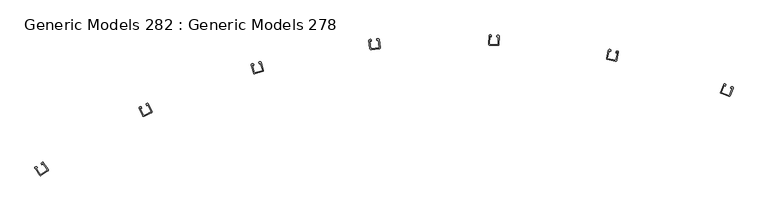
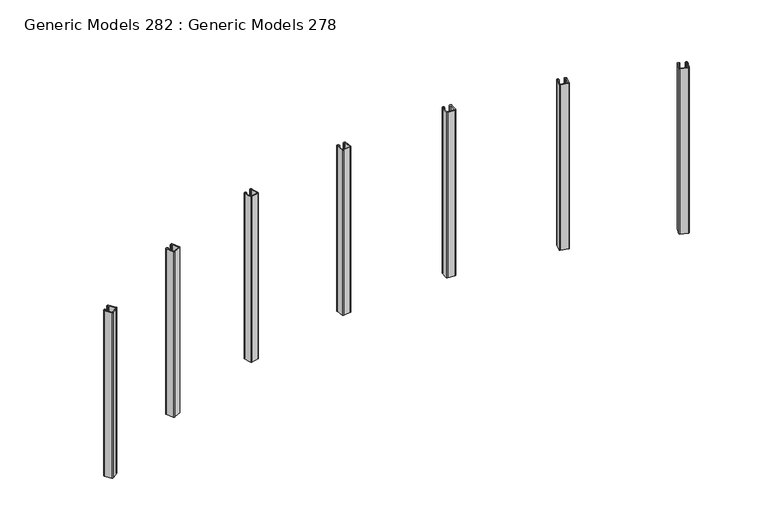
"""IFC4 building model written with IfcOpenShell, lengths in millimetres: proxy geometry, Generic Models 282 : Generic Models 278."""

from ifc_helpers import new_model, si_unit, point, frame, frame_2d, origin, place, context, project, spatial, polyline, circle_curve, trimmed, segment, composite_curve, outline, extrude, source, transform, mapped, element, save


def generic_models_282_generic_models_278_72c7d637(model_context):
    return source(origin(), model_context, "Body", "SweptSolid", [
        extrude(outline(composite_curve([segment(trimmed(circle_curve(frame_2d((271.5326409, -22367.9486308)), 3.9532868), [point((267.8419297, -22366.5318995))], [point((272.9493722, -22364.2579196))], False, "CARTESIAN"), True, "CONTINUOUS"), segment(polyline([(272.9493722, -22364.2579196), (274.3929251, -22364.8120477)]), True, "CONTINUOUS"), segment(trimmed(circle_curve(frame_2d((272.9503297, -22368.5701372)), 4.0254588), [point((274.3929251, -22364.8120477))], [point((276.7084192, -22370.0127326))], False, "CARTESIAN"), True, "CONTINUOUS"), segment(polyline([(276.7084192, -22370.0127326), (264.8013944, -22401.0315926)]), True, "CONTINUOUS"), segment(trimmed(circle_curve(frame_2d((261.0448118, -22399.5895756)), 4.0238446), [point((264.8013944, -22401.0315926))], [point((259.6027949, -22403.3461582))], False, "CARTESIAN"), True, "CONTINUOUS"), segment(polyline([(259.6027949, -22403.3461582), (228.5455312, -22391.4243917)]), True, "CONTINUOUS"), segment(trimmed(circle_curve(frame_2d((229.9733849, -22387.7047058)), 3.9843229), [point((228.5455312, -22391.4243917))], [point((226.253699, -22386.2768522))], False, "CARTESIAN"), True, "CONTINUOUS"), segment(polyline([(226.253699, -22386.2768522), (238.1797429, -22355.2084456)]), True, "CONTINUOUS"), segment(trimmed(circle_curve(frame_2d((241.9251825, -22356.6461852)), 4.0119089), [point((238.1797429, -22355.2084456))], [point((243.3629221, -22352.9007455))], False, "CARTESIAN"), True, "CONTINUOUS"), segment(polyline([(243.3629221, -22352.9007455), (244.734154, -22353.4271121)]), True, "CONTINUOUS"), segment(trimmed(circle_curve(frame_2d((243.2848054, -22357.2027942)), 4.0443029), [point((244.734154, -22353.4271121))], [point((247.0604875, -22358.6521427))], False, "CARTESIAN"), True, "CONTINUOUS"), segment(polyline([(247.0604875, -22358.6521427), (245.949745, -22361.5457259), (242.9856271, -22360.4079076), (244.0963696, -22357.5143245)]), True, "CONTINUOUS"), segment(trimmed(circle_curve(frame_2d((243.2848054, -22357.2027942)), 0.8693029), [point((244.0963696, -22357.5143245))], [point((243.5963357, -22356.39123))], True, "CARTESIAN"), True, "CONTINUOUS"), segment(polyline([(243.5963357, -22356.39123), (242.2251039, -22355.8648634)]), True, "CONTINUOUS"), segment(trimmed(circle_curve(frame_2d((241.9251825, -22356.6461852)), 0.8369089), [point((242.2251039, -22355.8648634))], [point((241.1438607, -22356.3462638))], True, "CARTESIAN"), True, "CONTINUOUS"), segment(polyline([(241.1438607, -22356.3462638), (229.2178168, -22387.4146704)]), True, "CONTINUOUS"), segment(trimmed(circle_curve(frame_2d((229.9733849, -22387.7047058)), 0.8093229), [point((229.2178168, -22387.4146704))], [point((229.6833495, -22388.4602738))], True, "CARTESIAN"), True, "CONTINUOUS"), segment(polyline([(229.6833495, -22388.4602738), (260.7406131, -22400.3820404)]), True, "CONTINUOUS"), segment(trimmed(circle_curve(frame_2d((261.0448118, -22399.5895756)), 0.8488446), [point((260.7406131, -22400.3820404))], [point((261.8372765, -22399.8937744))], True, "CARTESIAN"), True, "CONTINUOUS"), segment(polyline([(261.8372765, -22399.8937744), (273.7443013, -22368.8749143)]), True, "CONTINUOUS"), segment(trimmed(circle_curve(frame_2d((272.9503297, -22368.5701372)), 0.8504588), [point((273.7443013, -22368.8749143))], [point((273.2551068, -22367.7761655))], True, "CARTESIAN"), True, "CONTINUOUS"), segment(polyline([(273.2551068, -22367.7761655), (271.8115539, -22367.2220375)]), True, "CONTINUOUS"), segment(trimmed(circle_curve(frame_2d((271.5326409, -22367.9486308)), 0.7782868), [point((271.8115539, -22367.2220375))], [point((270.8060476, -22367.6697178))], True, "CARTESIAN"), True, "CONTINUOUS"), segment(polyline([(270.8060476, -22367.6697178), (269.6626878, -22370.6482718), (266.69857, -22369.5104535), (267.8419297, -22366.5318995)]), True, "CONTINUOUS")], self_intersect=False)), frame((0.0, 0.0, 203.2), z_axis=(0.0, 0.0, 1.0), x_axis=(1.0, 0.0, 0.0)), (0.0, 0.0, 1.0), 790.575),
        extrude(outline(composite_curve([segment(trimmed(circle_curve(frame_2d((-192.9016412, -22223.7493173)), 3.9532868), [point((-196.7670988, -22222.920635))], [point((-192.0729589, -22219.8838598))], False, "CARTESIAN"), True, "CONTINUOUS"), segment(polyline([(-192.0729589, -22219.8838598), (-190.5610572, -22220.2079834)]), True, "CONTINUOUS"), segment(trimmed(circle_curve(frame_2d((-191.4048681, -22224.1440095)), 4.0254588), [point((-190.5610572, -22220.2079834))], [point((-187.468842, -22224.9878204))], False, "CARTESIAN"), True, "CONTINUOUS"), segment(polyline([(-187.468842, -22224.9878204), (-194.4335648, -22257.4753496)]), True, "CONTINUOUS"), segment(trimmed(circle_curve(frame_2d((-198.3680126, -22256.6318771)), 4.0238446), [point((-194.4335648, -22257.4753496))], [point((-199.2114852, -22260.5663249))], False, "CARTESIAN"), True, "CONTINUOUS"), segment(polyline([(-199.2114852, -22260.5663249), (-231.7392362, -22253.5929793)]), True, "CONTINUOUS"), segment(trimmed(circle_curve(frame_2d((-230.9040482, -22249.6971751)), 3.9843229), [point((-231.7392362, -22253.5929793))], [point((-234.7998524, -22248.8619871))], False, "CARTESIAN"), True, "CONTINUOUS"), segment(polyline([(-234.7998524, -22248.8619871), (-227.8240048, -22216.3225654)]), True, "CONTINUOUS"), segment(trimmed(circle_curve(frame_2d((-223.9012275, -22217.163536)), 4.0119089), [point((-227.8240048, -22216.3225654))], [point((-223.060257, -22213.2407587))], False, "CARTESIAN"), True, "CONTINUOUS"), segment(polyline([(-223.060257, -22213.2407587), (-221.6241005, -22213.548644)]), True, "CONTINUOUS"), segment(trimmed(circle_curve(frame_2d((-222.4718615, -22217.5030956)), 4.0443029), [point((-221.6241005, -22213.548644))], [point((-218.5174099, -22218.3508565))], False, "CARTESIAN"), True, "CONTINUOUS"), segment(polyline([(-218.5174099, -22218.3508565), (-219.1671115, -22221.3814439), (-222.2715733, -22220.715905), (-221.6218717, -22217.6853176)]), True, "CONTINUOUS"), segment(trimmed(circle_curve(frame_2d((-222.4718615, -22217.5030956)), 0.8693029), [point((-221.6218717, -22217.6853176))], [point((-222.2896394, -22216.6531058))], True, "CARTESIAN"), True, "CONTINUOUS"), segment(polyline([(-222.2896394, -22216.6531058), (-223.7257959, -22216.3452205)]), True, "CONTINUOUS"), segment(trimmed(circle_curve(frame_2d((-223.9012275, -22217.163536)), 0.8369089), [point((-223.7257959, -22216.3452205))], [point((-224.719543, -22216.9881044))], True, "CARTESIAN"), True, "CONTINUOUS"), segment(polyline([(-224.719543, -22216.9881044), (-231.6953906, -22249.527526)]), True, "CONTINUOUS"), segment(trimmed(circle_curve(frame_2d((-230.9040482, -22249.6971751)), 0.8093229), [point((-231.6953906, -22249.527526))], [point((-231.0736973, -22250.4885175))], True, "CARTESIAN"), True, "CONTINUOUS"), segment(polyline([(-231.0736973, -22250.4885175), (-198.5459462, -22257.4618631)]), True, "CONTINUOUS"), segment(trimmed(circle_curve(frame_2d((-198.3680126, -22256.6318771)), 0.8488446), [point((-198.5459462, -22257.4618631))], [point((-197.5380266, -22256.8098106))], True, "CARTESIAN"), True, "CONTINUOUS"), segment(polyline([(-197.5380266, -22256.8098106), (-190.5733038, -22224.3222815)]), True, "CONTINUOUS"), segment(trimmed(circle_curve(frame_2d((-191.4048681, -22224.1440095)), 0.8504588), [point((-190.5733038, -22224.3222815))], [point((-191.2265962, -22223.3124452))], True, "CARTESIAN"), True, "CONTINUOUS"), segment(polyline([(-191.2265962, -22223.3124452), (-192.7384979, -22222.9883216)]), True, "CONTINUOUS"), segment(trimmed(circle_curve(frame_2d((-192.9016412, -22223.7493173)), 0.7782868), [point((-192.7384979, -22222.9883216))], [point((-193.662637, -22223.586174))], True, "CARTESIAN"), True, "CONTINUOUS"), segment(polyline([(-193.662637, -22223.586174), (-194.3314173, -22226.7057554), (-197.4358791, -22226.0402165), (-196.7670988, -22222.920635)]), True, "CONTINUOUS")], self_intersect=False)), frame((0.0, 0.0, 203.2), z_axis=(0.0, 0.0, 1.0), x_axis=(1.0, 0.0, 0.0)), (0.0, 0.0, 1.0), 790.575),
        extrude(outline(composite_curve([segment(trimmed(circle_curve(frame_2d((-675.3290548, -22159.8409899)), 3.9532868), [point((-679.2779529, -22159.6547646))], [point((-675.1428295, -22155.8920918))], False, "CARTESIAN"), True, "CONTINUOUS"), segment(polyline([(-675.1428295, -22155.8920918), (-673.5982915, -22155.9649304)]), True, "CONTINUOUS"), segment(trimmed(circle_curve(frame_2d((-673.7879166, -22159.9859204)), 4.0254588), [point((-673.5982915, -22155.9649304))], [point((-669.7669266, -22160.1755454))], False, "CARTESIAN"), True, "CONTINUOUS"), segment(polyline([(-669.7669266, -22160.1755454), (-671.3320713, -22193.3643574)]), True, "CONTINUOUS"), segment(trimmed(circle_curve(frame_2d((-675.3514489, -22193.1748083)), 4.0238446), [point((-671.3320713, -22193.3643574))], [point((-675.540998, -22197.194186))], False, "CARTESIAN"), True, "CONTINUOUS"), segment(polyline([(-675.540998, -22197.194186), (-708.7709001, -22195.6271036)]), True, "CONTINUOUS"), segment(trimmed(circle_curve(frame_2d((-708.5832127, -22191.6472037)), 3.9843229), [point((-708.7709001, -22195.6271036))], [point((-712.5631126, -22191.4595164))], False, "CARTESIAN"), True, "CONTINUOUS"), segment(polyline([(-712.5631126, -22191.4595164), (-710.9954679, -22158.2176919)]), True, "CONTINUOUS"), segment(trimmed(circle_curve(frame_2d((-706.9880127, -22158.4066787)), 4.0119089), [point((-710.9954679, -22158.2176919))], [point((-706.799026, -22154.3992235))], False, "CARTESIAN"), True, "CONTINUOUS"), segment(polyline([(-706.799026, -22154.3992235), (-705.3318683, -22154.4684129)]), True, "CONTINUOUS"), segment(trimmed(circle_curve(frame_2d((-705.5223811, -22158.5082261)), 4.0443029), [point((-705.3318683, -22154.4684129))], [point((-701.4825678, -22158.6987389))], False, "CARTESIAN"), True, "CONTINUOUS"), segment(polyline([(-701.4825678, -22158.6987389), (-701.6285718, -22161.7947452), (-704.8000471, -22161.6451822), (-704.6540432, -22158.5491759)]), True, "CONTINUOUS"), segment(trimmed(circle_curve(frame_2d((-705.5223811, -22158.5082261)), 0.8693029), [point((-704.6540432, -22158.5491759))], [point((-705.4814313, -22157.6398882))], True, "CARTESIAN"), True, "CONTINUOUS"), segment(polyline([(-705.4814313, -22157.6398882), (-706.9485889, -22157.5706988)]), True, "CONTINUOUS"), segment(trimmed(circle_curve(frame_2d((-706.9880127, -22158.4066787)), 0.8369089), [point((-706.9485889, -22157.5706988))], [point((-707.8239926, -22158.3672549))], True, "CARTESIAN"), True, "CONTINUOUS"), segment(polyline([(-707.8239926, -22158.3672549), (-709.3916372, -22191.6090794)]), True, "CONTINUOUS"), segment(trimmed(circle_curve(frame_2d((-708.5832127, -22191.6472037)), 0.8093229), [point((-709.3916372, -22191.6090794))], [point((-708.6213371, -22192.4556282))], True, "CARTESIAN"), True, "CONTINUOUS"), segment(polyline([(-708.6213371, -22192.4556282), (-675.391435, -22194.0227106)]), True, "CONTINUOUS"), segment(trimmed(circle_curve(frame_2d((-675.3514489, -22193.1748083)), 0.8488446), [point((-675.391435, -22194.0227106))], [point((-674.5035466, -22193.2147944))], True, "CARTESIAN"), True, "CONTINUOUS"), segment(polyline([(-674.5035466, -22193.2147944), (-672.938402, -22160.0259824)]), True, "CONTINUOUS"), segment(trimmed(circle_curve(frame_2d((-673.7879166, -22159.9859204)), 0.8504588), [point((-672.938402, -22160.0259824))], [point((-673.7478545, -22159.1364057))], True, "CARTESIAN"), True, "CONTINUOUS"), segment(polyline([(-673.7478545, -22159.1364057), (-675.2923925, -22159.0635672)]), True, "CONTINUOUS"), segment(trimmed(circle_curve(frame_2d((-675.3290548, -22159.8409899)), 0.7782868), [point((-675.2923925, -22159.0635672))], [point((-676.1064776, -22159.8043276))], True, "CARTESIAN"), True, "CONTINUOUS"), segment(polyline([(-676.1064776, -22159.8043276), (-676.256769, -22162.991249), (-679.4282443, -22162.841686), (-679.2779529, -22159.6547646)]), True, "CONTINUOUS")], self_intersect=False)), frame((0.0, 0.0, 203.2), z_axis=(0.0, 0.0, 1.0), x_axis=(1.0, 0.0, 0.0)), (0.0, 0.0, 1.0), 790.8083872),
        extrude(outline(composite_curve([segment(trimmed(circle_curve(frame_2d((-1639.18542, -22266.9192315)), 3.9532868), [point((-1642.9855632, -22268.0089051))], [point((-1640.2750935, -22263.1190884))], False, "CARTESIAN"), True, "CONTINUOUS"), segment(polyline([(-1640.2750935, -22263.1190884), (-1638.7887383, -22262.6928829)]), True, "CONTINUOUS"), segment(trimmed(circle_curve(frame_2d((-1637.6791715, -22266.5624022)), 4.0254588), [point((-1638.7887383, -22262.6928829))], [point((-1633.8096522, -22265.4528354))], False, "CARTESIAN"), True, "CONTINUOUS"), segment(polyline([(-1633.8096522, -22265.4528354), (-1624.6514091, -22297.3914249)]), True, "CONTINUOUS"), segment(trimmed(circle_curve(frame_2d((-1628.5193768, -22298.5005468)), 4.0238446), [point((-1624.6514091, -22297.3914249))], [point((-1627.4102549, -22302.3685145))], False, "CARTESIAN"), True, "CONTINUOUS"), segment(polyline([(-1627.4102549, -22302.3685145), (-1659.3883866, -22311.5380962)]), True, "CONTINUOUS"), segment(trimmed(circle_curve(frame_2d((-1660.4866149, -22307.7081192)), 3.9843229), [point((-1659.3883866, -22311.5380962))], [point((-1664.3165919, -22308.8063474))], False, "CARTESIAN"), True, "CONTINUOUS"), segment(polyline([(-1664.3165919, -22308.8063474), (-1673.4894636, -22276.8167423)]), True, "CONTINUOUS"), segment(trimmed(circle_curve(frame_2d((-1669.6329692, -22275.7109104)), 4.0119089), [point((-1673.4894636, -22276.8167423))], [point((-1670.7388012, -22271.854416))], False, "CARTESIAN"), True, "CONTINUOUS"), segment(polyline([(-1670.7388012, -22271.854416), (-1669.3269114, -22271.4495631)]), True, "CONTINUOUS"), segment(trimmed(circle_curve(frame_2d((-1668.2121504, -22275.3371966)), 4.0443029), [point((-1669.3269114, -22271.4495631))], [point((-1664.3245169, -22274.2224356))], False, "CARTESIAN"), True, "CONTINUOUS"), segment(polyline([(-1664.3245169, -22274.2224356), (-1663.4701935, -22277.2018154), (-1666.5221994, -22278.076964), (-1667.3765228, -22275.0975842)]), True, "CONTINUOUS"), segment(trimmed(circle_curve(frame_2d((-1668.2121504, -22275.3371966)), 0.8693029), [point((-1667.3765228, -22275.0975842))], [point((-1668.4517628, -22274.501569))], True, "CARTESIAN"), True, "CONTINUOUS"), segment(polyline([(-1668.4517628, -22274.501569), (-1669.8636526, -22274.9064219)]), True, "CONTINUOUS"), segment(trimmed(circle_curve(frame_2d((-1669.6329692, -22275.7109104)), 0.8369089), [point((-1669.8636526, -22274.9064219))], [point((-1670.4374577, -22275.9415937))], True, "CARTESIAN"), True, "CONTINUOUS"), segment(polyline([(-1670.4374577, -22275.9415937), (-1661.264586, -22307.9311988)]), True, "CONTINUOUS"), segment(trimmed(circle_curve(frame_2d((-1660.4866149, -22307.7081192)), 0.8093229), [point((-1661.264586, -22307.9311988))], [point((-1660.2635353, -22308.4860903))], True, "CARTESIAN"), True, "CONTINUOUS"), segment(polyline([(-1660.2635353, -22308.4860903), (-1628.2854035, -22299.3165086)]), True, "CONTINUOUS"), segment(trimmed(circle_curve(frame_2d((-1628.5193768, -22298.5005468)), 0.8488446), [point((-1628.2854035, -22299.3165086))], [point((-1627.703415, -22298.2665735))], True, "CARTESIAN"), True, "CONTINUOUS"), segment(polyline([(-1627.703415, -22298.2665735), (-1636.8616581, -22266.327984)]), True, "CONTINUOUS"), segment(trimmed(circle_curve(frame_2d((-1637.6791715, -22266.5624022)), 0.8504588), [point((-1636.8616581, -22266.327984))], [point((-1637.9135897, -22265.7448888))], True, "CARTESIAN"), True, "CONTINUOUS"), segment(polyline([(-1637.9135897, -22265.7448888), (-1639.3999449, -22266.1710943)]), True, "CONTINUOUS"), segment(trimmed(circle_curve(frame_2d((-1639.18542, -22266.9192315)), 0.7782868), [point((-1639.3999449, -22266.1710943))], [point((-1639.9335573, -22267.1337565))], True, "CARTESIAN"), True, "CONTINUOUS"), segment(polyline([(-1639.9335573, -22267.1337565), (-1639.0541464, -22270.2006265), (-1642.1061523, -22271.0757751), (-1642.9855632, -22268.0089051)]), True, "CONTINUOUS")], self_intersect=False)), frame((0.0, 0.0, 203.2), z_axis=(0.0, 0.0, 1.0), x_axis=(1.0, 0.0, 0.0)), (0.0, 0.0, 1.0), 790.575),
        extrude(outline(composite_curve([segment(trimmed(circle_curve(frame_2d((-2095.2333622, -22436.2715921)), 3.9532868), [point((-2098.8074598, -22437.9610603))], [point((-2096.9228304, -22432.6974945))], False, "CARTESIAN"), True, "CONTINUOUS"), segment(polyline([(-2096.9228304, -22432.6974945), (-2095.5248887, -22432.0366905)]), True, "CONTINUOUS"), segment(trimmed(circle_curve(frame_2d((-2093.8045773, -22435.6760375)), 4.0254588), [point((-2095.5248887, -22432.0366905))], [point((-2090.1652303, -22433.955726))], False, "CARTESIAN"), True, "CONTINUOUS"), segment(polyline([(-2090.1652303, -22433.955726), (-2075.9659676, -22463.9944985)]), True, "CONTINUOUS"), segment(trimmed(circle_curve(frame_2d((-2079.6038553, -22465.7141202)), 4.0238446), [point((-2075.9659676, -22463.9944985))], [point((-2077.8842336, -22469.3520079))], False, "CARTESIAN"), True, "CONTINUOUS"), segment(polyline([(-2077.8842336, -22469.3520079), (-2107.9601963, -22483.5688503)]), True, "CONTINUOUS"), segment(trimmed(circle_curve(frame_2d((-2109.6629281, -22479.9666935)), 3.9843229), [point((-2107.9601963, -22483.5688503))], [point((-2113.2650849, -22481.6694252))], False, "CARTESIAN"), True, "CONTINUOUS"), segment(polyline([(-2113.2650849, -22481.6694252), (-2127.4870281, -22451.5826717)]), True, "CONTINUOUS"), segment(trimmed(circle_curve(frame_2d((-2123.8599313, -22449.8681508)), 4.0119089), [point((-2127.4870281, -22451.5826717))], [point((-2125.5744521, -22446.241054))], False, "CARTESIAN"), True, "CONTINUOUS"), segment(polyline([(-2125.5744521, -22446.241054), (-2124.2465464, -22445.6133558)]), True, "CONTINUOUS"), segment(trimmed(circle_curve(frame_2d((-2122.5181817, -22449.2697395)), 4.0443029), [point((-2124.2465464, -22445.6133558))], [point((-2118.861798, -22447.5413749))], False, "CARTESIAN"), True, "CONTINUOUS"), segment(polyline([(-2118.861798, -22447.5413749), (-2117.5372249, -22450.3435309), (-2120.407687, -22451.7003921), (-2121.7322601, -22448.8982361)]), True, "CONTINUOUS"), segment(trimmed(circle_curve(frame_2d((-2122.5181817, -22449.2697395)), 0.8693029), [point((-2121.7322601, -22448.8982361))], [point((-2122.8896852, -22448.4838179))], True, "CARTESIAN"), True, "CONTINUOUS"), segment(polyline([(-2122.8896852, -22448.4838179), (-2124.2175909, -22449.1115161)]), True, "CONTINUOUS"), segment(trimmed(circle_curve(frame_2d((-2123.8599313, -22449.8681508)), 0.8369089), [point((-2124.2175909, -22449.1115161))], [point((-2124.6165661, -22450.2258105))], True, "CARTESIAN"), True, "CONTINUOUS"), segment(polyline([(-2124.6165661, -22450.2258105), (-2110.3946228, -22480.312564)]), True, "CONTINUOUS"), segment(trimmed(circle_curve(frame_2d((-2109.6629281, -22479.9666935)), 0.8093229), [point((-2110.3946228, -22480.312564))], [point((-2109.3170575, -22480.6983882))], True, "CARTESIAN"), True, "CONTINUOUS"), segment(polyline([(-2109.3170575, -22480.6983882), (-2079.2410949, -22466.4815458)]), True, "CONTINUOUS"), segment(trimmed(circle_curve(frame_2d((-2079.6038553, -22465.7141202)), 0.8488446), [point((-2079.2410949, -22466.4815458))], [point((-2078.8364297, -22465.3513598))], True, "CARTESIAN"), True, "CONTINUOUS"), segment(polyline([(-2078.8364297, -22465.3513598), (-2093.0356924, -22435.3125872)]), True, "CONTINUOUS"), segment(trimmed(circle_curve(frame_2d((-2093.8045773, -22435.6760375)), 0.8504588), [point((-2093.0356924, -22435.3125872))], [point((-2094.1680275, -22434.9071526))], True, "CARTESIAN"), True, "CONTINUOUS"), segment(polyline([(-2094.1680275, -22434.9071526), (-2095.5659692, -22435.5679566)]), True, "CONTINUOUS"), segment(trimmed(circle_curve(frame_2d((-2095.2333622, -22436.2715921)), 0.7782868), [point((-2095.5659692, -22435.5679566))], [point((-2095.9369977, -22436.604199))], True, "CARTESIAN"), True, "CONTINUOUS"), segment(polyline([(-2095.9369977, -22436.604199), (-2094.5735282, -22439.4886412), (-2097.4439903, -22440.8455024), (-2098.8074598, -22437.9610603)]), True, "CONTINUOUS")], self_intersect=False)), frame((0.0, 0.0, 203.2), z_axis=(0.0, 0.0, 1.0), x_axis=(1.0, 0.0, 0.0)), (0.0, 0.0, 1.0), 790.575),
        extrude(outline(composite_curve([segment(trimmed(circle_curve(frame_2d((-2519.7783276, -22674.4696616)), 3.9532868), [point((-2523.0284988, -22676.7201869))], [point((-2522.0288528, -22671.2194905))], False, "CARTESIAN"), True, "CONTINUOUS"), segment(polyline([(-2522.0288528, -22671.2194905), (-2520.7576089, -22670.3392395)]), True, "CONTINUOUS"), segment(trimmed(circle_curve(frame_2d((-2518.4659977, -22673.6487464)), 4.0254588), [point((-2520.7576089, -22670.3392395))], [point((-2515.1564907, -22671.3571352))], False, "CARTESIAN"), True, "CONTINUOUS"), segment(polyline([(-2515.1564907, -22671.3571352), (-2496.241782, -22698.6734436)]), True, "CONTINUOUS"), segment(trimmed(circle_curve(frame_2d((-2499.5499619, -22700.964136)), 4.0238446), [point((-2496.241782, -22698.6734436))], [point((-2497.2592695, -22704.2723159))], False, "CARTESIAN"), True, "CONTINUOUS"), segment(polyline([(-2497.2592695, -22704.2723159), (-2524.6093976, -22723.2104424)]), True, "CONTINUOUS"), segment(trimmed(circle_curve(frame_2d((-2526.877591, -22719.934755)), 3.9843229), [point((-2524.6093976, -22723.2104424))], [point((-2530.1532784, -22722.2029485))], False, "CARTESIAN"), True, "CONTINUOUS"), segment(polyline([(-2530.1532784, -22722.2029485), (-2549.0981997, -22694.8430076)]), True, "CONTINUOUS"), segment(trimmed(circle_curve(frame_2d((-2545.7998327, -22692.55911)), 4.0119089), [point((-2549.0981997, -22694.8430076))], [point((-2548.0837303, -22689.260743))], False, "CARTESIAN"), True, "CONTINUOUS"), segment(polyline([(-2548.0837303, -22689.260743), (-2546.8761748, -22688.4245919)]), True, "CONTINUOUS"), segment(trimmed(circle_curve(frame_2d((-2544.573836, -22691.7495915)), 4.0443029), [point((-2546.8761748, -22688.4245919))], [point((-2541.2488364, -22689.4472526))], False, "CARTESIAN"), True, "CONTINUOUS"), segment(polyline([(-2541.2488364, -22689.4472526), (-2539.4843847, -22691.9954446), (-2542.094692, -22693.8029071), (-2543.8591438, -22691.2547151)]), True, "CONTINUOUS"), segment(trimmed(circle_curve(frame_2d((-2544.573836, -22691.7495915)), 0.8693029), [point((-2543.8591438, -22691.2547151))], [point((-2545.0687123, -22691.0348993))], True, "CARTESIAN"), True, "CONTINUOUS"), segment(polyline([(-2545.0687123, -22691.0348993), (-2546.2762678, -22691.8710503)]), True, "CONTINUOUS"), segment(trimmed(circle_curve(frame_2d((-2545.7998327, -22692.55911)), 0.8369089), [point((-2546.2762678, -22691.8710503))], [point((-2546.4878923, -22693.0355451))], True, "CARTESIAN"), True, "CONTINUOUS"), segment(polyline([(-2546.4878923, -22693.0355451), (-2527.5429711, -22720.395486)]), True, "CONTINUOUS"), segment(trimmed(circle_curve(frame_2d((-2526.877591, -22719.934755)), 0.8093229), [point((-2527.5429711, -22720.395486))], [point((-2526.4168601, -22720.6001351))], True, "CARTESIAN"), True, "CONTINUOUS"), segment(polyline([(-2526.4168601, -22720.6001351), (-2499.066732, -22701.6620085)]), True, "CONTINUOUS"), segment(trimmed(circle_curve(frame_2d((-2499.5499619, -22700.964136)), 0.8488446), [point((-2499.066732, -22701.6620085))], [point((-2498.8520893, -22700.4809061))], True, "CARTESIAN"), True, "CONTINUOUS"), segment(polyline([(-2498.8520893, -22700.4809061), (-2517.7667981, -22673.1645976)]), True, "CONTINUOUS"), segment(trimmed(circle_curve(frame_2d((-2518.4659977, -22673.6487464)), 0.8504588), [point((-2517.7667981, -22673.1645976))], [point((-2518.9501464, -22672.9495468))], True, "CARTESIAN"), True, "CONTINUOUS"), segment(polyline([(-2518.9501464, -22672.9495468), (-2520.2213903, -22673.8297978)]), True, "CONTINUOUS"), segment(trimmed(circle_curve(frame_2d((-2519.7783276, -22674.4696616)), 0.7782868), [point((-2520.2213903, -22673.8297978))], [point((-2520.4181914, -22674.9127244))], True, "CARTESIAN"), True, "CONTINUOUS"), segment(polyline([(-2520.4181914, -22674.9127244), (-2518.601926, -22677.5357447), (-2521.2122334, -22679.3432072), (-2523.0284988, -22676.7201869)]), True, "CONTINUOUS")], self_intersect=False)), frame((0.0, 0.0, 203.2), z_axis=(0.0, 0.0, 1.0), x_axis=(1.0, 0.0, 0.0)), (0.0, 0.0, 1.0), 790.575),
        extrude(outline(composite_curve([segment(trimmed(circle_curve(frame_2d((-1161.7816613, -22173.0789113)), 3.9532868), [point((-1165.7054809, -22173.5606958))], [point((-1162.2634458, -22169.1550918))], False, "CARTESIAN"), True, "CONTINUOUS"), segment(polyline([(-1162.2634458, -22169.1550918), (-1160.7287169, -22168.9666507)]), True, "CONTINUOUS"), segment(trimmed(circle_curve(frame_2d((-1160.2381369, -22172.9621043)), 4.0254588), [point((-1160.7287169, -22168.9666507))], [point((-1156.2426833, -22172.4715243))], False, "CARTESIAN"), True, "CONTINUOUS"), segment(polyline([(-1156.2426833, -22172.4715243), (-1152.1934894, -22205.4495616)]), True, "CONTINUOUS"), segment(trimmed(circle_curve(frame_2d((-1156.187341, -22205.9399449)), 4.0238446), [point((-1152.1934894, -22205.4495616))], [point((-1155.6969576, -22209.9337964))], False, "CARTESIAN"), True, "CONTINUOUS"), segment(polyline([(-1155.6969576, -22209.9337964), (-1188.7158242, -22213.9880035)]), True, "CONTINUOUS"), segment(trimmed(circle_curve(frame_2d((-1189.201391, -22210.0333791)), 3.9843229), [point((-1188.7158242, -22213.9880035))], [point((-1193.1560154, -22210.5189459))], False, "CARTESIAN"), True, "CONTINUOUS"), segment(polyline([(-1193.1560154, -22210.5189459), (-1197.211677, -22177.4882326)]), True, "CONTINUOUS"), segment(trimmed(circle_curve(frame_2d((-1193.2296722, -22176.9993039)), 4.0119089), [point((-1197.211677, -22177.4882326))], [point((-1193.718601, -22173.0172992))], False, "CARTESIAN"), True, "CONTINUOUS"), segment(polyline([(-1193.718601, -22173.0172992), (-1192.2607609, -22172.8382989)]), True, "CONTINUOUS"), segment(trimmed(circle_curve(frame_2d((-1191.7678844, -22176.8524562)), 4.0443029), [point((-1192.2607609, -22172.8382989))], [point((-1187.7537271, -22176.3595797))], False, "CARTESIAN"), True, "CONTINUOUS"), segment(polyline([(-1187.7537271, -22176.3595797), (-1187.3759995, -22179.435924), (-1190.5273335, -22179.8228591), (-1190.9050611, -22176.7465148)]), True, "CONTINUOUS"), segment(trimmed(circle_curve(frame_2d((-1191.7678844, -22176.8524562)), 0.8693029), [point((-1190.9050611, -22176.7465148))], [point((-1191.8738257, -22175.989633))], True, "CARTESIAN"), True, "CONTINUOUS"), segment(polyline([(-1191.8738257, -22175.989633), (-1193.3316658, -22176.1686332)]), True, "CONTINUOUS"), segment(trimmed(circle_curve(frame_2d((-1193.2296722, -22176.9993039)), 0.8369089), [point((-1193.3316658, -22176.1686332))], [point((-1194.060343, -22177.1012975))], True, "CARTESIAN"), True, "CONTINUOUS"), segment(polyline([(-1194.060343, -22177.1012975), (-1190.0046813, -22210.1320107)]), True, "CONTINUOUS"), segment(trimmed(circle_curve(frame_2d((-1189.201391, -22210.0333791)), 0.8093229), [point((-1190.0046813, -22210.1320107))], [point((-1189.1027593, -22210.8366694))], True, "CARTESIAN"), True, "CONTINUOUS"), segment(polyline([(-1189.1027593, -22210.8366694), (-1156.0838928, -22206.7824624)]), True, "CONTINUOUS"), segment(trimmed(circle_curve(frame_2d((-1156.187341, -22205.9399449)), 0.8488446), [point((-1156.0838928, -22206.7824624))], [point((-1155.3448235, -22205.8364968))], True, "CARTESIAN"), True, "CONTINUOUS"), segment(polyline([(-1155.3448235, -22205.8364968), (-1159.3940173, -22172.8584595)]), True, "CONTINUOUS"), segment(trimmed(circle_curve(frame_2d((-1160.2381369, -22172.9621043)), 0.8504588), [point((-1159.3940173, -22172.8584595))], [point((-1160.3417817, -22172.1179848))], True, "CARTESIAN"), True, "CONTINUOUS"), segment(polyline([(-1160.3417817, -22172.1179848), (-1161.8765106, -22172.3064258)]), True, "CONTINUOUS"), segment(trimmed(circle_curve(frame_2d((-1161.7816613, -22173.0789113)), 0.7782868), [point((-1161.8765106, -22172.3064258))], [point((-1162.5541469, -22173.1737606))], True, "CARTESIAN"), True, "CONTINUOUS"), segment(polyline([(-1162.5541469, -22173.1737606), (-1162.1653272, -22176.3404426), (-1165.3166613, -22176.7273778), (-1165.7054809, -22173.5606958)]), True, "CONTINUOUS")], self_intersect=False)), frame((0.0, 0.0, 203.2), z_axis=(0.0, 0.0, 1.0), x_axis=(1.0, 0.0, 0.0)), (0.0, 0.0, 1.0), 790.575),
    ])


if __name__ == "__main__":
    model = new_model("IFC4")
    model_context = context("Model", 3, world=origin())
    ifc_project = project(units=[si_unit("LENGTHUNIT", "METRE", prefix="MILLI")], contexts=[model_context])
    site = spatial("IfcSite", under=ifc_project)
    building = spatial("IfcBuilding", under=site)
    placement = place(None, origin())
    generic_models_282_generic_models_278_shape = generic_models_282_generic_models_278_72c7d637(model_context)
    element("IfcBuildingElementProxy", 1, Name="Generic Models 282 : Generic Models 278", ObjectType="Generic Models 282 : Generic Models 278", at=placement, inside=building, context=model_context, shape_type="MappedRepresentation", body=[
        mapped(generic_models_282_generic_models_278_shape, transform((0.0, 0.0, 0.0), x_axis=(1.0, 0.0, 0.0), y_axis=(0.0, 1.0, 0.0), z_axis=(0.0, 0.0, 1.0))),
    ])
    save(model, "model.ifc")

# Revit data of these elements
# Element 1 (IfcBuildingElementProxy, "Generic Models 282 : Generic Models 278")
#   Materials on its faces: "UNISTRUT P1000, 1 5/8\" X 1 5/8\", PERFORATED CHANNEL OR ALUM. CHANNEL"
# Materials
#   "UNISTRUT P1000, 1 5/8\" X 1 5/8\", PERFORATED CHANNEL OR ALUM. CHANNEL": class "Metal", colour RGB 244 244 244, transparency 0, Description = "Aluminum 6061", Cost = 0
